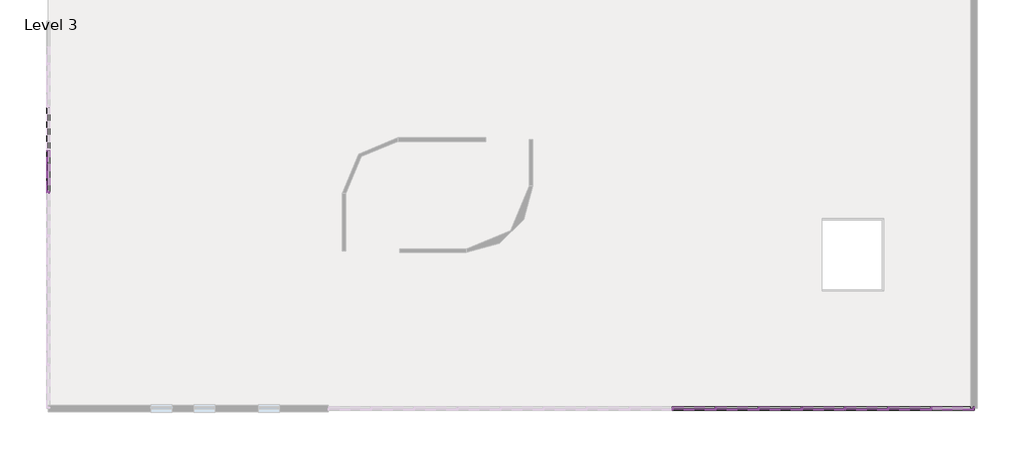
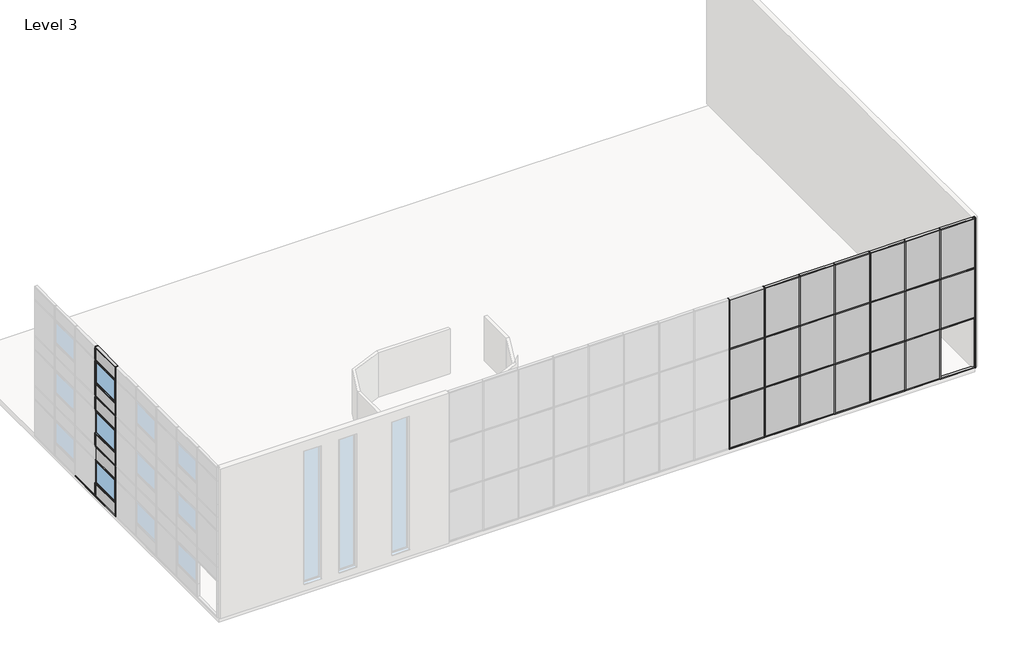
# One storey, part 3 of 5: 77 members, 26 plates, 3 windows.
"""IFC4 building model written with IfcOpenShell, lengths in millimetres."""

import ifcopenshell
import ifcopenshell.guid

model = None  # the IFC model being written
_history = None  # IfcOwnerHistory: only IFC2X3 demands one
_inside = {}  # id of a spatial element -> (the spatial element, [elements in it])
_under = {}  # id of a project, library or spatial element -> (it, [spatial elements below it])
_declared = {}  # id of a project -> (the project, [libraries it declares])
_typed = {}  # id of a type object -> (the type object, [elements of that type])
_made_of = {}  # id of a material, layer set ... -> (it, [elements and type objects made of it])


def new_model(schema):
    """Start an empty IFC model of exactly this schema.

    Asked for "IFC4X3", IfcOpenShell would pick the latest addendum, in which some entities
    have other attributes; the version numbers below select the first issue.
    IFC2X3 requires an IfcOwnerHistory on every rooted entity: one is made here for all.
    """
    global model, _history
    if schema == "IFC4X3":
        model = ifcopenshell.file(schema_version=(4, 3, 0, 0))
    else:
        model = ifcopenshell.file(schema=schema)
    _inside.clear()
    _under.clear()
    _declared.clear()
    _typed.clear()
    _made_of.clear()
    _history = None
    if model.schema == "IFC2X3":
        org = make("IfcOrganization", Name="unknown")
        user = make(
            "IfcPersonAndOrganization",
            ThePerson=make("IfcPerson", FamilyName="unknown"),
            TheOrganization=org,
        )
        app = make(
            "IfcApplication",
            ApplicationDeveloper=org,
            Version="unknown",
            ApplicationFullName="unknown",
            ApplicationIdentifier="unknown",
        )
        _history = make(
            "IfcOwnerHistory",
            OwningUser=user,
            OwningApplication=app,
            ChangeAction="ADDED",
            CreationDate=0,
        )
    return model


def make(cls, **values):
    """One entity of the class cls with the attributes given. An attribute that is None is left unset."""
    return model.create_entity(
        cls, **{name: value for name, value in values.items() if value is not None}
    )


def rooted(cls, **values):
    """An entity with a GlobalId (a new one), such as an element, a storey or a relation."""
    return make(cls, GlobalId=ifcopenshell.guid.new(), OwnerHistory=_history, **values)


def si_unit(unit_type, name, prefix=None):
    """IfcSIUnit, for example si_unit("LENGTHUNIT", "METRE", prefix="MILLI")."""
    return make("IfcSIUnit", UnitType=unit_type, Prefix=prefix, Name=name)


def assignment(units):
    """IfcUnitAssignment: the units of a project."""
    return None if units is None else make("IfcUnitAssignment", Units=units)


def point(xyz):
    """IfcCartesianPoint."""
    return None if xyz is None else make("IfcCartesianPoint", Coordinates=xyz)


def direction(xyz):
    """IfcDirection."""
    return None if xyz is None else make("IfcDirection", DirectionRatios=xyz)


def frame(location, z_axis=None, x_axis=None):
    """IfcAxis2Placement3D, a coordinate frame: its origin and axes. An axis left out is left unset."""
    return make(
        "IfcAxis2Placement3D",
        Location=point(location),
        Axis=direction(z_axis),
        RefDirection=direction(x_axis),
    )


def origin():
    """The frame at (0, 0, 0) with its axes left unset."""
    return frame((0.0, 0.0, 0.0))


def origin_with_axes():
    """The frame at (0, 0, 0) with the z axis (0, 0, 1) and the x axis (1, 0, 0) written out."""
    return frame((0.0, 0.0, 0.0), z_axis=(0.0, 0.0, 1.0), x_axis=(1.0, 0.0, 0.0))


def place(relative_to, where):
    """IfcLocalPlacement: puts the frame where relative to a parent placement (None: the world)."""
    return make(
        "IfcLocalPlacement", PlacementRelTo=relative_to, RelativePlacement=where
    )


def context(
    kind, dimensions, precision=None, world=None, true_north=None, identifier=None
):
    """IfcGeometricRepresentationContext, for example the 3D "Model" context."""
    return make(
        "IfcGeometricRepresentationContext",
        ContextIdentifier=identifier,
        ContextType=kind,
        CoordinateSpaceDimension=dimensions,
        Precision=precision,
        WorldCoordinateSystem=world,
        TrueNorth=true_north,
    )


def project(units=None, contexts=None):
    """IfcProject with its units and contexts."""
    return rooted(
        "IfcProject",
        Name="project",
        RepresentationContexts=contexts,
        UnitsInContext=assignment(units),
    )


def spatial(cls, under=None, at=None, **own):
    """A site, building, storey or space (cls), placed at a placement, below another one or the project."""
    s = rooted(cls, ObjectPlacement=at, **own)
    if under is not None:
        _under.setdefault(under.id(), (under, []))[1].append(s)
    return s


def polyline(points):
    """IfcPolyline through the points."""
    return make("IfcPolyline", Points=[point(p) for p in points])


def outline(outer, holes=None, kind="AREA"):
    """IfcArbitraryClosedProfileDef: a profile drawn as a closed curve; with holes, ...WithVoids."""
    if holes is None:
        return make("IfcArbitraryClosedProfileDef", ProfileType=kind, OuterCurve=outer)
    return make(
        "IfcArbitraryProfileDefWithVoids",
        ProfileType=kind,
        OuterCurve=outer,
        InnerCurves=holes,
    )


def extrude(swept, where, along, depth):
    """IfcExtrudedAreaSolid: the profile swept, set in the frame where, extruded along a direction by depth."""
    return make(
        "IfcExtrudedAreaSolid",
        SweptArea=swept,
        Position=where,
        ExtrudedDirection=direction(along),
        Depth=depth,
    )


def shape(context_of_items, identifier, shape_type, items):
    """IfcShapeRepresentation: the items that make up one representation, for example the "Body"."""
    return make(
        "IfcShapeRepresentation",
        ContextOfItems=context_of_items,
        RepresentationIdentifier=identifier,
        RepresentationType=shape_type,
        Items=items,
    )


def source(mapping_origin, context_of_items, identifier, shape_type, items):
    """IfcRepresentationMap: a shape defined once, which mapped items show again and again."""
    return make(
        "IfcRepresentationMap",
        MappingOrigin=mapping_origin,
        MappedRepresentation=shape(context_of_items, identifier, shape_type, items),
    )


def transform(
    local_origin,
    x_axis=None,
    y_axis=None,
    z_axis=None,
    scale=None,
    scale2=None,
    scale3=None,
    uniform=True,
):
    """IfcCartesianTransformationOperator3D, or its non-uniform kind. x_axis, y_axis, z_axis: its Axis1, 2, 3."""
    if uniform:
        return make(
            "IfcCartesianTransformationOperator3D",
            Axis1=direction(x_axis),
            Axis2=direction(y_axis),
            LocalOrigin=point(local_origin),
            Scale=scale,
            Axis3=direction(z_axis),
        )
    return make(
        "IfcCartesianTransformationOperator3DnonUniform",
        Axis1=direction(x_axis),
        Axis2=direction(y_axis),
        LocalOrigin=point(local_origin),
        Scale=scale,
        Axis3=direction(z_axis),
        Scale2=scale2,
        Scale3=scale3,
    )


def mapped(mapping_source, mapping_target):
    """IfcMappedItem: shows the shape of a source again, moved by a transform."""
    return make(
        "IfcMappedItem", MappingSource=mapping_source, MappingTarget=mapping_target
    )


def made_of(thing, what):
    """Note that an element or type object is made of a material, layer set ...; save() writes the relation."""
    if what is not None:
        _made_of.setdefault(what.id(), (what, []))[1].append(thing)
    return thing


def element(
    cls,
    number,
    at=None,
    inside=None,
    cuts=None,
    type_object=None,
    material=None,
    context=None,
    identifier="Body",
    shape_type=None,
    held_by="IfcProductDefinitionShape",
    body=None,
    shapes=None,
    **own,
):
    """One element of the class cls, such as IfcWall. Its Tag is "e" and its number.

    at: its placement. inside: the storey or other place that contains it. cuts: it is an
    opening in that element (IfcRelVoidsElement). A single representation is given by context,
    identifier, shape_type and body (its items); several are given by shapes. held_by: the class
    of the entity that holds the representations. save() writes the other relations.
    """
    e = rooted(cls, Tag="e%d" % number, ObjectPlacement=at, **own)
    if body is not None:
        shapes = [shape(context, identifier, shape_type, body)]
    if shapes is not None:
        e.Representation = make(held_by, Representations=shapes)
    if inside is not None:
        _inside.setdefault(inside.id(), (inside, []))[1].append(e)
    if cuts is not None:
        rooted(
            "IfcRelVoidsElement", RelatingBuildingElement=cuts, RelatedOpeningElement=e
        )
    if type_object is not None:
        _typed.setdefault(type_object.id(), (type_object, []))[1].append(e)
    return made_of(e, material)


def aggregate(whole, parts):
    """IfcRelAggregates: a whole, such as a stair, and the parts it consists of."""
    return rooted("IfcRelAggregates", RelatingObject=whole, RelatedObjects=parts)


def save(model, path):
    """Write the relations noted so far, then the file.

    IfcRelAggregates (storeys below a building ...), IfcRelContainedInSpatialStructure (elements
    in a storey), IfcRelDefinesByType, IfcRelAssociatesMaterial and IfcRelDeclares: one each for
    every whole, place, type object, material and project.
    """
    for whole, parts in _under.values():
        aggregate(whole, parts)
    for where, things in _inside.values():
        rooted(
            "IfcRelContainedInSpatialStructure",
            RelatedElements=things,
            RelatingStructure=where,
        )
    for kind, things in _typed.values():
        rooted("IfcRelDefinesByType", RelatedObjects=things, RelatingType=kind)
    for what, things in _made_of.values():
        rooted("IfcRelAssociatesMaterial", RelatedObjects=things, RelatingMaterial=what)
    for by, libraries in _declared.values():
        rooted("IfcRelDeclares", RelatingContext=by, RelatedDefinitions=libraries)
    model.write(path)


def rectangular_mullion_50_x_150mm_0967fd3c(model_context):
    return source(origin(), model_context, "Body", "SweptSolid", [
        extrude(outline(polyline([(0.0, 75.0), (0.0, -75.0), (-50.0, -75.0), (-50.0, 75.0), (0.0, 75.0)])), frame((0.0, 0.0, -1950.0000003), z_axis=(0.0, 0.0, 1.0), x_axis=(1.0, 0.0, 0.0)), (0.0, 0.0, 1.0), 1950.0000003),
    ])


def rectangular_mullion_50_x_150mm_f1645b81(model_context):
    return source(origin(), model_context, "Body", "SweptSolid", [
        extrude(outline(polyline([(25.0, 75.0), (25.0, -75.0), (-25.0, -75.0), (-25.0, 75.0), (25.0, 75.0)])), frame((0.0, 0.0, -1950.0000003), z_axis=(0.0, 0.0, 1.0), x_axis=(1.0, 0.0, 0.0)), (0.0, 0.0, 1.0), 1950.0000003),
    ])


def rectangular_mullion_50_x_150mm_14f10ac7(model_context):
    return source(origin(), model_context, "Body", "SweptSolid", [
        extrude(outline(polyline([(25.0, 75.0), (25.0, -75.0), (-25.0, -75.0), (-25.0, 75.0), (25.0, 75.0)])), frame((0.0, 0.0, -800.0), z_axis=(0.0, 0.0, 1.0), x_axis=(1.0, 0.0, 0.0)), (0.0, 0.0, 1.0), 800.0),
    ])


def rectangular_mullion_50_x_150mm_6270d9f9(model_context):
    return source(origin(), model_context, "Body", "SweptSolid", [
        extrude(outline(polyline([(25.0, 75.0), (25.0, -75.0), (-25.0, -75.0), (-25.0, 75.0), (25.0, 75.0)])), frame((0.0, 0.0, -775.0), z_axis=(0.0, 0.0, 1.0), x_axis=(1.0, 0.0, 0.0)), (0.0, 0.0, 1.0), 775.0),
    ])


def rectangular_mullion_50_x_150mm_80d7b263(model_context):
    return source(origin(), model_context, "Body", "SweptSolid", [
        extrude(outline(polyline([(25.0, 75.0), (25.0, -75.0), (-25.0, -75.0), (-25.0, 75.0), (25.0, 75.0)])), frame((0.0, 0.0, -1400.0), z_axis=(0.0, 0.0, 1.0), x_axis=(1.0, 0.0, 0.0)), (0.0, 0.0, 1.0), 1400.0),
    ])


def rectangular_mullion_50_x_150mm_9c26cac3(model_context):
    return source(origin(), model_context, "Body", "SweptSolid", [
        extrude(outline(polyline([(25.0, 75.0), (25.0, -75.0), (-25.0, -75.0), (-25.0, 75.0), (25.0, 75.0)])), frame((0.0, 0.0, -825.0), z_axis=(0.0, 0.0, 1.0), x_axis=(1.0, 0.0, 0.0)), (0.0, 0.0, 1.0), 825.0),
    ])


def rectangular_mullion_50_x_150mm_6c7cb899(model_context):
    return source(origin(), model_context, "Body", "SweptSolid", [
        extrude(outline(polyline([(25.0, 75.0), (25.0, -75.0), (-25.0, -75.0), (-25.0, 75.0), (25.0, 75.0)])), frame((0.0, 0.0, -3000.0), z_axis=(0.0, 0.0, 1.0), x_axis=(1.0, 0.0, 0.0)), (0.0, 0.0, 1.0), 3000.0),
    ])


def rectangular_mullion_50_x_150mm_68c91185(model_context):
    return source(origin(), model_context, "Body", "SweptSolid", [
        extrude(outline(polyline([(0.0, 75.0), (0.0, -75.0), (-50.0, -75.0), (-50.0, 75.0), (0.0, 75.0)])), frame((0.0, 0.0, -3000.0), z_axis=(0.0, 0.0, 1.0), x_axis=(1.0, 0.0, 0.0)), (0.0, 0.0, 1.0), 3000.0),
    ])


def rectangular_mullion_50_x_150mm_7828da58(model_context):
    return source(origin(), model_context, "Body", "SweptSolid", [
        extrude(outline(polyline([(0.0, 75.0), (0.0, -75.0), (-50.0, -75.0), (-50.0, 75.0), (0.0, 75.0)])), frame((0.0, 0.0, -1923.3666669), z_axis=(0.0, 0.0, 1.0), x_axis=(1.0, 0.0, 0.0)), (0.0, 0.0, 1.0), 1923.3666669),
    ])


def rectangular_mullion_50_x_150mm_2c1a111c(model_context):
    return source(origin(), model_context, "Body", "SweptSolid", [
        extrude(outline(polyline([(0.0, 75.0), (0.0, -75.0), (-50.0, -75.0), (-50.0, 75.0), (0.0, 75.0)])), frame((0.0, 0.0, -1948.3666666), z_axis=(0.0, 0.0, 1.0), x_axis=(1.0, 0.0, 0.0)), (0.0, 0.0, 1.0), 1948.3666666),
    ])


def rectangular_mullion_50_x_150mm_6ba4331c(model_context):
    return source(origin(), model_context, "Body", "SweptSolid", [
        extrude(outline(polyline([(25.0, 75.0), (25.0, -75.0), (-25.0, -75.0), (-25.0, 75.0), (25.0, 75.0)])), frame((0.0, 0.0, -1923.3666669), z_axis=(0.0, 0.0, 1.0), x_axis=(1.0, 0.0, 0.0)), (0.0, 0.0, 1.0), 1923.3666669),
    ])


def rectangular_mullion_50_x_150mm_825cde95(model_context):
    return source(origin(), model_context, "Body", "SweptSolid", [
        extrude(outline(polyline([(25.0, 75.0), (25.0, -75.0), (-25.0, -75.0), (-25.0, 75.0), (25.0, 75.0)])), frame((0.0, 0.0, -1948.3666666), z_axis=(0.0, 0.0, 1.0), x_axis=(1.0, 0.0, 0.0)), (0.0, 0.0, 1.0), 1948.3666666),
    ])


def system_panel_glazed_bc1ebc0c(model_context):
    return source(origin(), model_context, "Body", "SweptSolid", [
        extrude(outline(polyline([(975.0000002, 24.5), (-975.0000002, 24.5), (-975.0000002, 49.5), (975.0000002, 49.5), (975.0000002, 24.5)])), origin_with_axes(), (0.0, 0.0, 1.0), 725.0),
    ])


def system_panel_glazed_d82c9dbb(model_context):
    return source(origin(), model_context, "Body", "SweptSolid", [
        extrude(outline(polyline([(975.0000002, 24.5), (-975.0000002, 24.5), (-975.0000002, 49.5), (975.0000002, 49.5), (975.0000002, 24.5)])), origin_with_axes(), (0.0, 0.0, 1.0), 775.0),
    ])


def system_panel_glazed_19a6ddb1(model_context):
    return source(origin(), model_context, "Body", "SweptSolid", [
        extrude(outline(polyline([(961.6833335, 24.5), (-961.6833335, 24.5), (-961.6833335, 49.5), (961.6833335, 49.5), (961.6833335, 24.5)])), origin_with_axes(), (0.0, 0.0, 1.0), 2925.0),
    ])


def system_panel_glazed_e38ee6be(model_context):
    return source(origin(), model_context, "Body", "SweptSolid", [
        extrude(outline(polyline([(974.1833333, 24.5), (-974.1833333, 24.5), (-974.1833333, 49.5), (974.1833333, 49.5), (974.1833333, 24.5)])), origin_with_axes(), (0.0, 0.0, 1.0), 2925.0),
    ])


def system_panel_glazed_cab7de13(model_context):
    return source(origin(), model_context, "Body", "SweptSolid", [
        extrude(outline(polyline([(961.6833335, 24.5), (-961.6833335, 24.5), (-961.6833335, 49.5), (961.6833335, 49.5), (961.6833335, 24.5)])), origin_with_axes(), (0.0, 0.0, 1.0), 2950.0),
    ])


def system_panel_glazed_2cf92cf8(model_context):
    return source(origin(), model_context, "Body", "SweptSolid", [
        extrude(outline(polyline([(974.1833333, 24.5), (-974.1833333, 24.5), (-974.1833333, 49.5), (974.1833333, 49.5), (974.1833333, 24.5)])), origin_with_axes(), (0.0, 0.0, 1.0), 2950.0),
    ])


def m_curtain_wall_awning_m_curtain_wall_awning_db665c81(model_context):
    return source(origin(), model_context, "Body", "SweptSolid", [
        extrude(outline(polyline([(900.0, 44.05), (-900.0, 44.05), (-900.0, 56.75), (900.0, 56.75), (900.0, 44.05)])), frame((0.0, 0.0, 75.0), z_axis=(0.0, 0.0, 1.0), x_axis=(1.0, 0.0, 0.0)), (0.0, 0.0, 1.0), 1200.0),
        extrude(outline(polyline([(1350.0, -975.0), (0.0, -975.0), (0.0, 975.0), (1350.0, 975.0), (1350.0, -975.0)]), holes=[polyline([(1275.0, -900.0), (1275.0, 900.0), (75.0, 900.0), (75.0, -900.0), (1275.0, -900.0)])]), frame((0.0, 25.0, 0.0), z_axis=(0.0, 1.0, 0.0), x_axis=(0.0, 0.0, 1.0)), (0.0, 0.0, 1.0), 50.0),
    ])


model = new_model("IFC4")

# Units and contexts
model_context = context("Model", 3, world=origin())
ifc_project = project(units=[si_unit("LENGTHUNIT", "METRE", prefix="MILLI")], contexts=[model_context])

# Site, building, storey
site = spatial("IfcSite", under=ifc_project)
building = spatial("IfcBuilding", under=site)
storey = spatial("IfcBuildingStorey", under=building, Name="Level 3", Elevation=6000.0)

# Members
placement = place(None, origin())
rectangular_mullion_50_x_150mm_shape = rectangular_mullion_50_x_150mm_0967fd3c(model_context)
element("IfcMember", 1, ObjectType="Rectangular Mullion : 50 x 150mm", at=placement, inside=storey, context=model_context, shape_type="MappedRepresentation", body=[
    mapped(rectangular_mullion_50_x_150mm_shape, transform((-6732.0028633, 48.7577233, 6000.0), x_axis=(0.0, 0.0, -1.0), y_axis=(1.0, 0.0, 0.0), z_axis=(0.0, -1.0, 0.0))),
])
element("IfcMember", 2, ObjectType="Rectangular Mullion : 50 x 150mm", at=placement, inside=storey, context=model_context, shape_type="MappedRepresentation", body=[
    mapped(rectangular_mullion_50_x_150mm_shape, transform((-6732.0028633, 2048.7577233, 6000.0), x_axis=(0.0, 0.0, -1.0), y_axis=(1.0, 0.0, 0.0), z_axis=(0.0, -1.0, 0.0))),
])
rectangular_mullion_50_x_150mm_2_shape = rectangular_mullion_50_x_150mm_f1645b81(model_context)
element("IfcMember", 3, ObjectType="Rectangular Mullion : 50 x 150mm", at=placement, inside=storey, context=model_context, shape_type="MappedRepresentation", body=[
    mapped(rectangular_mullion_50_x_150mm_2_shape, transform((-6732.0028633, 1998.7577233, 14200.0), x_axis=(0.0, 0.0, 1.0), y_axis=(1.0, 0.0, 0.0), z_axis=(0.0, 1.0, 0.0))),
])
element("IfcMember", 4, ObjectType="Rectangular Mullion : 50 x 150mm", at=placement, inside=storey, context=model_context, shape_type="MappedRepresentation", body=[
    mapped(rectangular_mullion_50_x_150mm_2_shape, transform((-6732.0028633, 1998.7577233, 9025.0), x_axis=(0.0, 0.0, 1.0), y_axis=(1.0, 0.0, 0.0), z_axis=(0.0, 1.0, 0.0))),
])
element("IfcMember", 5, ObjectType="Rectangular Mullion : 50 x 150mm", at=placement, inside=storey, context=model_context, shape_type="MappedRepresentation", body=[
    mapped(rectangular_mullion_50_x_150mm_2_shape, transform((-6732.0028633, 1998.7577233, 12025.0), x_axis=(0.0, 0.0, 1.0), y_axis=(1.0, 0.0, 0.0), z_axis=(0.0, 1.0, 0.0))),
])
element("IfcMember", 6, ObjectType="Rectangular Mullion : 50 x 150mm", at=placement, inside=storey, context=model_context, shape_type="MappedRepresentation", body=[
    mapped(rectangular_mullion_50_x_150mm_2_shape, transform((-6732.0028633, 1998.7577233, 12800.0), x_axis=(0.0, 0.0, 1.0), y_axis=(1.0, 0.0, 0.0), z_axis=(0.0, 1.0, 0.0))),
])
element("IfcMember", 7, ObjectType="Rectangular Mullion : 50 x 150mm", at=placement, inside=storey, context=model_context, shape_type="MappedRepresentation", body=[
    mapped(rectangular_mullion_50_x_150mm_2_shape, transform((-6732.0028633, 1998.7577233, 11200.0), x_axis=(0.0, 0.0, 1.0), y_axis=(1.0, 0.0, 0.0), z_axis=(0.0, 1.0, 0.0))),
])
element("IfcMember", 8, ObjectType="Rectangular Mullion : 50 x 150mm", at=placement, inside=storey, context=model_context, shape_type="MappedRepresentation", body=[
    mapped(rectangular_mullion_50_x_150mm_2_shape, transform((-6732.0028633, 1998.7577233, 9800.0), x_axis=(0.0, 0.0, 1.0), y_axis=(1.0, 0.0, 0.0), z_axis=(0.0, 1.0, 0.0))),
])
element("IfcMember", 9, ObjectType="Rectangular Mullion : 50 x 150mm", at=placement, inside=storey, context=model_context, shape_type="MappedRepresentation", body=[
    mapped(rectangular_mullion_50_x_150mm_2_shape, transform((-6732.0028633, 1998.7577233, 8200.0), x_axis=(0.0, 0.0, 1.0), y_axis=(1.0, 0.0, 0.0), z_axis=(0.0, 1.0, 0.0))),
])
element("IfcMember", 10, ObjectType="Rectangular Mullion : 50 x 150mm", at=placement, inside=storey, context=model_context, shape_type="MappedRepresentation", body=[
    mapped(rectangular_mullion_50_x_150mm_2_shape, transform((-6732.0028633, 1998.7577233, 6800.0), x_axis=(0.0, 0.0, 1.0), y_axis=(1.0, 0.0, 0.0), z_axis=(0.0, 1.0, 0.0))),
])
rectangular_mullion_50_x_150mm_3_shape = rectangular_mullion_50_x_150mm_14f10ac7(model_context)
element("IfcMember", 11, ObjectType="Rectangular Mullion : 50 x 150mm", at=placement, inside=storey, context=model_context, shape_type="MappedRepresentation", body=[
    mapped(rectangular_mullion_50_x_150mm_3_shape, transform((-6732.0028633, 23.7577233, 6000.0), x_axis=(0.0, 1.0, 0.0), y_axis=(1.0, 0.0, 0.0), z_axis=(0.0, 0.0, -1.0))),
])
element("IfcMember", 12, ObjectType="Rectangular Mullion : 50 x 150mm", at=placement, inside=storey, context=model_context, shape_type="MappedRepresentation", body=[
    mapped(rectangular_mullion_50_x_150mm_3_shape, transform((-6732.0028633, 2023.7577233, 6000.0), x_axis=(0.0, 1.0, 0.0), y_axis=(1.0, 0.0, 0.0), z_axis=(0.0, 0.0, -1.0))),
])
element("IfcMember", 13, ObjectType="Rectangular Mullion : 50 x 150mm", at=placement, inside=storey, context=model_context, shape_type="MappedRepresentation", body=[
    mapped(rectangular_mullion_50_x_150mm_shape, transform((-6732.0028633, 1998.7577233, 15000.0), x_axis=(0.0, 0.0, 1.0), y_axis=(1.0, 0.0, 0.0), z_axis=(0.0, 1.0, 0.0))),
])
element("IfcMember", 14, ObjectType="Rectangular Mullion : 50 x 150mm", at=placement, inside=storey, context=model_context, shape_type="MappedRepresentation", body=[
    mapped(rectangular_mullion_50_x_150mm_3_shape, transform((-6732.0028633, 23.7577233, 14200.0), x_axis=(0.0, 1.0, 0.0), y_axis=(1.0, 0.0, 0.0), z_axis=(0.0, 0.0, -1.0))),
])
element("IfcMember", 15, ObjectType="Rectangular Mullion : 50 x 150mm", at=placement, inside=storey, context=model_context, shape_type="MappedRepresentation", body=[
    mapped(rectangular_mullion_50_x_150mm_3_shape, transform((-6732.0028633, 2023.7577233, 14200.0), x_axis=(0.0, 1.0, 0.0), y_axis=(1.0, 0.0, 0.0), z_axis=(0.0, 0.0, -1.0))),
])
rectangular_mullion_50_x_150mm_4_shape = rectangular_mullion_50_x_150mm_6270d9f9(model_context)
element("IfcMember", 16, ObjectType="Rectangular Mullion : 50 x 150mm", at=placement, inside=storey, context=model_context, shape_type="MappedRepresentation", body=[
    mapped(rectangular_mullion_50_x_150mm_4_shape, transform((-6732.0028633, 23.7577233, 9025.0), x_axis=(0.0, 1.0, 0.0), y_axis=(1.0, 0.0, 0.0), z_axis=(0.0, 0.0, -1.0))),
])
element("IfcMember", 17, ObjectType="Rectangular Mullion : 50 x 150mm", at=placement, inside=storey, context=model_context, shape_type="MappedRepresentation", body=[
    mapped(rectangular_mullion_50_x_150mm_4_shape, transform((-6732.0028633, 23.7577233, 12025.0), x_axis=(0.0, 1.0, 0.0), y_axis=(1.0, 0.0, 0.0), z_axis=(0.0, 0.0, -1.0))),
])
element("IfcMember", 18, ObjectType="Rectangular Mullion : 50 x 150mm", at=placement, inside=storey, context=model_context, shape_type="MappedRepresentation", body=[
    mapped(rectangular_mullion_50_x_150mm_4_shape, transform((-6732.0028633, 2023.7577233, 9025.0), x_axis=(0.0, 1.0, 0.0), y_axis=(1.0, 0.0, 0.0), z_axis=(0.0, 0.0, -1.0))),
])
element("IfcMember", 19, ObjectType="Rectangular Mullion : 50 x 150mm", at=placement, inside=storey, context=model_context, shape_type="MappedRepresentation", body=[
    mapped(rectangular_mullion_50_x_150mm_4_shape, transform((-6732.0028633, 2023.7577233, 12025.0), x_axis=(0.0, 1.0, 0.0), y_axis=(1.0, 0.0, 0.0), z_axis=(0.0, 0.0, -1.0))),
])
rectangular_mullion_50_x_150mm_5_shape = rectangular_mullion_50_x_150mm_80d7b263(model_context)
element("IfcMember", 20, ObjectType="Rectangular Mullion : 50 x 150mm", at=placement, inside=storey, context=model_context, shape_type="MappedRepresentation", body=[
    mapped(rectangular_mullion_50_x_150mm_5_shape, transform((-6732.0028633, 23.7577233, 12800.0), x_axis=(0.0, 1.0, 0.0), y_axis=(1.0, 0.0, 0.0), z_axis=(0.0, 0.0, -1.0))),
])
element("IfcMember", 21, ObjectType="Rectangular Mullion : 50 x 150mm", at=placement, inside=storey, context=model_context, shape_type="MappedRepresentation", body=[
    mapped(rectangular_mullion_50_x_150mm_5_shape, transform((-6732.0028633, 23.7577233, 9800.0), x_axis=(0.0, 1.0, 0.0), y_axis=(1.0, 0.0, 0.0), z_axis=(0.0, 0.0, -1.0))),
])
element("IfcMember", 22, ObjectType="Rectangular Mullion : 50 x 150mm", at=placement, inside=storey, context=model_context, shape_type="MappedRepresentation", body=[
    mapped(rectangular_mullion_50_x_150mm_5_shape, transform((-6732.0028633, 23.7577233, 6800.0), x_axis=(0.0, 1.0, 0.0), y_axis=(1.0, 0.0, 0.0), z_axis=(0.0, 0.0, -1.0))),
])
element("IfcMember", 23, ObjectType="Rectangular Mullion : 50 x 150mm", at=placement, inside=storey, context=model_context, shape_type="MappedRepresentation", body=[
    mapped(rectangular_mullion_50_x_150mm_5_shape, transform((-6732.0028633, 2023.7577233, 12800.0), x_axis=(0.0, 1.0, 0.0), y_axis=(1.0, 0.0, 0.0), z_axis=(0.0, 0.0, -1.0))),
])
rectangular_mullion_50_x_150mm_6_shape = rectangular_mullion_50_x_150mm_9c26cac3(model_context)
element("IfcMember", 24, ObjectType="Rectangular Mullion : 50 x 150mm", at=placement, inside=storey, context=model_context, shape_type="MappedRepresentation", body=[
    mapped(rectangular_mullion_50_x_150mm_6_shape, transform((-6732.0028633, 23.7577233, 11200.0), x_axis=(0.0, 1.0, 0.0), y_axis=(1.0, 0.0, 0.0), z_axis=(0.0, 0.0, -1.0))),
])
element("IfcMember", 25, ObjectType="Rectangular Mullion : 50 x 150mm", at=placement, inside=storey, context=model_context, shape_type="MappedRepresentation", body=[
    mapped(rectangular_mullion_50_x_150mm_6_shape, transform((-6732.0028633, 23.7577233, 8200.0), x_axis=(0.0, 1.0, 0.0), y_axis=(1.0, 0.0, 0.0), z_axis=(0.0, 0.0, -1.0))),
])
element("IfcMember", 26, ObjectType="Rectangular Mullion : 50 x 150mm", at=placement, inside=storey, context=model_context, shape_type="MappedRepresentation", body=[
    mapped(rectangular_mullion_50_x_150mm_6_shape, transform((-6732.0028633, 2023.7577233, 11200.0), x_axis=(0.0, 1.0, 0.0), y_axis=(1.0, 0.0, 0.0), z_axis=(0.0, 0.0, -1.0))),
])
rectangular_mullion_50_x_150mm_7_shape = rectangular_mullion_50_x_150mm_6c7cb899(model_context)
element("IfcMember", 27, ObjectType="Rectangular Mullion : 50 x 150mm", at=placement, inside=storey, context=model_context, shape_type="MappedRepresentation", body=[
    mapped(rectangular_mullion_50_x_150mm_7_shape, transform((34245.1304697, -10001.242277, 6000.0), x_axis=(-1.0, 0.0, 0.0), y_axis=(0.0, 1.0, 0.0), z_axis=(0.0, 0.0, -1.0))),
])
element("IfcMember", 28, ObjectType="Rectangular Mullion : 50 x 150mm", at=placement, inside=storey, context=model_context, shape_type="MappedRepresentation", body=[
    mapped(rectangular_mullion_50_x_150mm_7_shape, transform((32246.7638031, -10001.242277, 6000.0), x_axis=(-1.0, 0.0, 0.0), y_axis=(0.0, 1.0, 0.0), z_axis=(0.0, 0.0, -1.0))),
])
element("IfcMember", 29, ObjectType="Rectangular Mullion : 50 x 150mm", at=placement, inside=storey, context=model_context, shape_type="MappedRepresentation", body=[
    mapped(rectangular_mullion_50_x_150mm_7_shape, transform((30248.3971365, -10001.242277, 6000.0), x_axis=(-1.0, 0.0, 0.0), y_axis=(0.0, 1.0, 0.0), z_axis=(0.0, 0.0, -1.0))),
])
element("IfcMember", 30, ObjectType="Rectangular Mullion : 50 x 150mm", at=placement, inside=storey, context=model_context, shape_type="MappedRepresentation", body=[
    mapped(rectangular_mullion_50_x_150mm_7_shape, transform((28250.0304699, -10001.242277, 6000.0), x_axis=(-1.0, 0.0, 0.0), y_axis=(0.0, 1.0, 0.0), z_axis=(0.0, 0.0, -1.0))),
])
element("IfcMember", 31, ObjectType="Rectangular Mullion : 50 x 150mm", at=placement, inside=storey, context=model_context, shape_type="MappedRepresentation", body=[
    mapped(rectangular_mullion_50_x_150mm_7_shape, transform((26251.6638032, -10001.242277, 6000.0), x_axis=(-1.0, 0.0, 0.0), y_axis=(0.0, 1.0, 0.0), z_axis=(0.0, 0.0, -1.0))),
])
element("IfcMember", 32, ObjectType="Rectangular Mullion : 50 x 150mm", at=placement, inside=storey, context=model_context, shape_type="MappedRepresentation", body=[
    mapped(rectangular_mullion_50_x_150mm_7_shape, transform((24253.2971366, -10001.242277, 6000.0), x_axis=(-1.0, 0.0, 0.0), y_axis=(0.0, 1.0, 0.0), z_axis=(0.0, 0.0, -1.0))),
])
element("IfcMember", 33, ObjectType="Rectangular Mullion : 50 x 150mm", at=placement, inside=storey, context=model_context, shape_type="MappedRepresentation", body=[
    mapped(rectangular_mullion_50_x_150mm_7_shape, transform((22254.93047, -10001.242277, 6000.0), x_axis=(-1.0, 0.0, 0.0), y_axis=(0.0, 1.0, 0.0), z_axis=(0.0, 0.0, -1.0))),
])
rectangular_mullion_50_x_150mm_8_shape = rectangular_mullion_50_x_150mm_68c91185(model_context)
element("IfcMember", 34, ObjectType="Rectangular Mullion : 50 x 150mm", at=placement, inside=storey, context=model_context, shape_type="MappedRepresentation", body=[
    mapped(rectangular_mullion_50_x_150mm_8_shape, transform((36243.4971367, -10001.242277, 9000.0), x_axis=(1.0, 0.0, 0.0), y_axis=(0.0, 1.0, 0.0), z_axis=(0.0, 0.0, 1.0))),
])
rectangular_mullion_50_x_150mm_9_shape = rectangular_mullion_50_x_150mm_7828da58(model_context)
element("IfcMember", 35, ObjectType="Rectangular Mullion : 50 x 150mm", at=placement, inside=storey, context=model_context, shape_type="MappedRepresentation", body=[
    mapped(rectangular_mullion_50_x_150mm_9_shape, transform((34270.1304697, -10001.242277, 15000.0), x_axis=(0.0, 0.0, 1.0), y_axis=(0.0, 1.0, 0.0), z_axis=(-1.0, 0.0, 0.0))),
])
element("IfcMember", 36, ObjectType="Rectangular Mullion : 50 x 150mm", at=placement, inside=storey, context=model_context, shape_type="MappedRepresentation", body=[
    mapped(rectangular_mullion_50_x_150mm_9_shape, transform((36193.4971367, -10001.242277, 6000.0), x_axis=(0.0, 0.0, -1.0), y_axis=(0.0, 1.0, 0.0), z_axis=(1.0, 0.0, 0.0))),
])
rectangular_mullion_50_x_150mm_10_shape = rectangular_mullion_50_x_150mm_2c1a111c(model_context)
element("IfcMember", 37, ObjectType="Rectangular Mullion : 50 x 150mm", at=placement, inside=storey, context=model_context, shape_type="MappedRepresentation", body=[
    mapped(rectangular_mullion_50_x_150mm_10_shape, transform((32271.7638031, -10001.242277, 15000.0), x_axis=(0.0, 0.0, 1.0), y_axis=(0.0, 1.0, 0.0), z_axis=(-1.0, 0.0, 0.0))),
])
element("IfcMember", 38, ObjectType="Rectangular Mullion : 50 x 150mm", at=placement, inside=storey, context=model_context, shape_type="MappedRepresentation", body=[
    mapped(rectangular_mullion_50_x_150mm_10_shape, transform((30273.3971365, -10001.242277, 15000.0), x_axis=(0.0, 0.0, 1.0), y_axis=(0.0, 1.0, 0.0), z_axis=(-1.0, 0.0, 0.0))),
])
element("IfcMember", 39, ObjectType="Rectangular Mullion : 50 x 150mm", at=placement, inside=storey, context=model_context, shape_type="MappedRepresentation", body=[
    mapped(rectangular_mullion_50_x_150mm_10_shape, transform((28275.0304699, -10001.242277, 15000.0), x_axis=(0.0, 0.0, 1.0), y_axis=(0.0, 1.0, 0.0), z_axis=(-1.0, 0.0, 0.0))),
])
element("IfcMember", 40, ObjectType="Rectangular Mullion : 50 x 150mm", at=placement, inside=storey, context=model_context, shape_type="MappedRepresentation", body=[
    mapped(rectangular_mullion_50_x_150mm_10_shape, transform((26276.6638032, -10001.242277, 15000.0), x_axis=(0.0, 0.0, 1.0), y_axis=(0.0, 1.0, 0.0), z_axis=(-1.0, 0.0, 0.0))),
])
element("IfcMember", 41, ObjectType="Rectangular Mullion : 50 x 150mm", at=placement, inside=storey, context=model_context, shape_type="MappedRepresentation", body=[
    mapped(rectangular_mullion_50_x_150mm_10_shape, transform((24278.2971366, -10001.242277, 15000.0), x_axis=(0.0, 0.0, 1.0), y_axis=(0.0, 1.0, 0.0), z_axis=(-1.0, 0.0, 0.0))),
])
element("IfcMember", 42, ObjectType="Rectangular Mullion : 50 x 150mm", at=placement, inside=storey, context=model_context, shape_type="MappedRepresentation", body=[
    mapped(rectangular_mullion_50_x_150mm_10_shape, transform((34220.1304697, -10001.242277, 6000.0), x_axis=(0.0, 0.0, -1.0), y_axis=(0.0, 1.0, 0.0), z_axis=(1.0, 0.0, 0.0))),
])
element("IfcMember", 43, ObjectType="Rectangular Mullion : 50 x 150mm", at=placement, inside=storey, context=model_context, shape_type="MappedRepresentation", body=[
    mapped(rectangular_mullion_50_x_150mm_10_shape, transform((32221.7638031, -10001.242277, 6000.0), x_axis=(0.0, 0.0, -1.0), y_axis=(0.0, 1.0, 0.0), z_axis=(1.0, 0.0, 0.0))),
])
element("IfcMember", 44, ObjectType="Rectangular Mullion : 50 x 150mm", at=placement, inside=storey, context=model_context, shape_type="MappedRepresentation", body=[
    mapped(rectangular_mullion_50_x_150mm_10_shape, transform((30223.3971365, -10001.242277, 6000.0), x_axis=(0.0, 0.0, -1.0), y_axis=(0.0, 1.0, 0.0), z_axis=(1.0, 0.0, 0.0))),
])
element("IfcMember", 45, ObjectType="Rectangular Mullion : 50 x 150mm", at=placement, inside=storey, context=model_context, shape_type="MappedRepresentation", body=[
    mapped(rectangular_mullion_50_x_150mm_10_shape, transform((28225.0304699, -10001.242277, 6000.0), x_axis=(0.0, 0.0, -1.0), y_axis=(0.0, 1.0, 0.0), z_axis=(1.0, 0.0, 0.0))),
])
element("IfcMember", 46, ObjectType="Rectangular Mullion : 50 x 150mm", at=placement, inside=storey, context=model_context, shape_type="MappedRepresentation", body=[
    mapped(rectangular_mullion_50_x_150mm_10_shape, transform((26226.6638032, -10001.242277, 6000.0), x_axis=(0.0, 0.0, -1.0), y_axis=(0.0, 1.0, 0.0), z_axis=(1.0, 0.0, 0.0))),
])
element("IfcMember", 47, ObjectType="Rectangular Mullion : 50 x 150mm", at=placement, inside=storey, context=model_context, shape_type="MappedRepresentation", body=[
    mapped(rectangular_mullion_50_x_150mm_10_shape, transform((24228.2971366, -10001.242277, 6000.0), x_axis=(0.0, 0.0, -1.0), y_axis=(0.0, 1.0, 0.0), z_axis=(1.0, 0.0, 0.0))),
])
rectangular_mullion_50_x_150mm_11_shape = rectangular_mullion_50_x_150mm_6ba4331c(model_context)
element("IfcMember", 48, ObjectType="Rectangular Mullion : 50 x 150mm", at=placement, inside=storey, context=model_context, shape_type="MappedRepresentation", body=[
    mapped(rectangular_mullion_50_x_150mm_11_shape, transform((34270.1304697, -10001.242277, 9000.0), x_axis=(0.0, 0.0, 1.0), y_axis=(0.0, 1.0, 0.0), z_axis=(-1.0, 0.0, 0.0))),
])
element("IfcMember", 49, ObjectType="Rectangular Mullion : 50 x 150mm", at=placement, inside=storey, context=model_context, shape_type="MappedRepresentation", body=[
    mapped(rectangular_mullion_50_x_150mm_11_shape, transform((34270.1304697, -10001.242277, 12000.0), x_axis=(0.0, 0.0, 1.0), y_axis=(0.0, 1.0, 0.0), z_axis=(-1.0, 0.0, 0.0))),
])
rectangular_mullion_50_x_150mm_12_shape = rectangular_mullion_50_x_150mm_825cde95(model_context)
element("IfcMember", 50, ObjectType="Rectangular Mullion : 50 x 150mm", at=placement, inside=storey, context=model_context, shape_type="MappedRepresentation", body=[
    mapped(rectangular_mullion_50_x_150mm_12_shape, transform((32271.7638031, -10001.242277, 9000.0), x_axis=(0.0, 0.0, 1.0), y_axis=(0.0, 1.0, 0.0), z_axis=(-1.0, 0.0, 0.0))),
])
element("IfcMember", 51, ObjectType="Rectangular Mullion : 50 x 150mm", at=placement, inside=storey, context=model_context, shape_type="MappedRepresentation", body=[
    mapped(rectangular_mullion_50_x_150mm_12_shape, transform((30273.3971365, -10001.242277, 9000.0), x_axis=(0.0, 0.0, 1.0), y_axis=(0.0, 1.0, 0.0), z_axis=(-1.0, 0.0, 0.0))),
])
element("IfcMember", 52, ObjectType="Rectangular Mullion : 50 x 150mm", at=placement, inside=storey, context=model_context, shape_type="MappedRepresentation", body=[
    mapped(rectangular_mullion_50_x_150mm_12_shape, transform((28275.0304699, -10001.242277, 9000.0), x_axis=(0.0, 0.0, 1.0), y_axis=(0.0, 1.0, 0.0), z_axis=(-1.0, 0.0, 0.0))),
])
element("IfcMember", 53, ObjectType="Rectangular Mullion : 50 x 150mm", at=placement, inside=storey, context=model_context, shape_type="MappedRepresentation", body=[
    mapped(rectangular_mullion_50_x_150mm_12_shape, transform((26276.6638032, -10001.242277, 9000.0), x_axis=(0.0, 0.0, 1.0), y_axis=(0.0, 1.0, 0.0), z_axis=(-1.0, 0.0, 0.0))),
])
element("IfcMember", 54, ObjectType="Rectangular Mullion : 50 x 150mm", at=placement, inside=storey, context=model_context, shape_type="MappedRepresentation", body=[
    mapped(rectangular_mullion_50_x_150mm_12_shape, transform((24278.2971366, -10001.242277, 9000.0), x_axis=(0.0, 0.0, 1.0), y_axis=(0.0, 1.0, 0.0), z_axis=(-1.0, 0.0, 0.0))),
])
element("IfcMember", 55, ObjectType="Rectangular Mullion : 50 x 150mm", at=placement, inside=storey, context=model_context, shape_type="MappedRepresentation", body=[
    mapped(rectangular_mullion_50_x_150mm_12_shape, transform((22279.93047, -10001.242277, 9000.0), x_axis=(0.0, 0.0, 1.0), y_axis=(0.0, 1.0, 0.0), z_axis=(-1.0, 0.0, 0.0))),
])
element("IfcMember", 56, ObjectType="Rectangular Mullion : 50 x 150mm", at=placement, inside=storey, context=model_context, shape_type="MappedRepresentation", body=[
    mapped(rectangular_mullion_50_x_150mm_12_shape, transform((32271.7638031, -10001.242277, 12000.0), x_axis=(0.0, 0.0, 1.0), y_axis=(0.0, 1.0, 0.0), z_axis=(-1.0, 0.0, 0.0))),
])
element("IfcMember", 57, ObjectType="Rectangular Mullion : 50 x 150mm", at=placement, inside=storey, context=model_context, shape_type="MappedRepresentation", body=[
    mapped(rectangular_mullion_50_x_150mm_12_shape, transform((30273.3971365, -10001.242277, 12000.0), x_axis=(0.0, 0.0, 1.0), y_axis=(0.0, 1.0, 0.0), z_axis=(-1.0, 0.0, 0.0))),
])
element("IfcMember", 58, ObjectType="Rectangular Mullion : 50 x 150mm", at=placement, inside=storey, context=model_context, shape_type="MappedRepresentation", body=[
    mapped(rectangular_mullion_50_x_150mm_12_shape, transform((28275.0304699, -10001.242277, 12000.0), x_axis=(0.0, 0.0, 1.0), y_axis=(0.0, 1.0, 0.0), z_axis=(-1.0, 0.0, 0.0))),
])
element("IfcMember", 59, ObjectType="Rectangular Mullion : 50 x 150mm", at=placement, inside=storey, context=model_context, shape_type="MappedRepresentation", body=[
    mapped(rectangular_mullion_50_x_150mm_12_shape, transform((26276.6638032, -10001.242277, 12000.0), x_axis=(0.0, 0.0, 1.0), y_axis=(0.0, 1.0, 0.0), z_axis=(-1.0, 0.0, 0.0))),
])
element("IfcMember", 60, ObjectType="Rectangular Mullion : 50 x 150mm", at=placement, inside=storey, context=model_context, shape_type="MappedRepresentation", body=[
    mapped(rectangular_mullion_50_x_150mm_12_shape, transform((24278.2971366, -10001.242277, 12000.0), x_axis=(0.0, 0.0, 1.0), y_axis=(0.0, 1.0, 0.0), z_axis=(-1.0, 0.0, 0.0))),
])
element("IfcMember", 61, ObjectType="Rectangular Mullion : 50 x 150mm", at=placement, inside=storey, context=model_context, shape_type="MappedRepresentation", body=[
    mapped(rectangular_mullion_50_x_150mm_12_shape, transform((22279.93047, -10001.242277, 12000.0), x_axis=(0.0, 0.0, 1.0), y_axis=(0.0, 1.0, 0.0), z_axis=(-1.0, 0.0, 0.0))),
])
element("IfcMember", 62, ObjectType="Rectangular Mullion : 50 x 150mm", at=placement, inside=storey, context=model_context, shape_type="MappedRepresentation", body=[
    mapped(rectangular_mullion_50_x_150mm_7_shape, transform((34245.1304697, -10001.242277, 9000.0), x_axis=(-1.0, 0.0, 0.0), y_axis=(0.0, 1.0, 0.0), z_axis=(0.0, 0.0, -1.0))),
])
element("IfcMember", 63, ObjectType="Rectangular Mullion : 50 x 150mm", at=placement, inside=storey, context=model_context, shape_type="MappedRepresentation", body=[
    mapped(rectangular_mullion_50_x_150mm_7_shape, transform((32246.7638031, -10001.242277, 9000.0), x_axis=(-1.0, 0.0, 0.0), y_axis=(0.0, 1.0, 0.0), z_axis=(0.0, 0.0, -1.0))),
])
element("IfcMember", 64, ObjectType="Rectangular Mullion : 50 x 150mm", at=placement, inside=storey, context=model_context, shape_type="MappedRepresentation", body=[
    mapped(rectangular_mullion_50_x_150mm_7_shape, transform((30248.3971365, -10001.242277, 9000.0), x_axis=(-1.0, 0.0, 0.0), y_axis=(0.0, 1.0, 0.0), z_axis=(0.0, 0.0, -1.0))),
])
element("IfcMember", 65, ObjectType="Rectangular Mullion : 50 x 150mm", at=placement, inside=storey, context=model_context, shape_type="MappedRepresentation", body=[
    mapped(rectangular_mullion_50_x_150mm_7_shape, transform((28250.0304699, -10001.242277, 9000.0), x_axis=(-1.0, 0.0, 0.0), y_axis=(0.0, 1.0, 0.0), z_axis=(0.0, 0.0, -1.0))),
])
element("IfcMember", 66, ObjectType="Rectangular Mullion : 50 x 150mm", at=placement, inside=storey, context=model_context, shape_type="MappedRepresentation", body=[
    mapped(rectangular_mullion_50_x_150mm_7_shape, transform((26251.6638032, -10001.242277, 9000.0), x_axis=(-1.0, 0.0, 0.0), y_axis=(0.0, 1.0, 0.0), z_axis=(0.0, 0.0, -1.0))),
])
element("IfcMember", 67, ObjectType="Rectangular Mullion : 50 x 150mm", at=placement, inside=storey, context=model_context, shape_type="MappedRepresentation", body=[
    mapped(rectangular_mullion_50_x_150mm_7_shape, transform((24253.2971366, -10001.242277, 9000.0), x_axis=(-1.0, 0.0, 0.0), y_axis=(0.0, 1.0, 0.0), z_axis=(0.0, 0.0, -1.0))),
])
element("IfcMember", 68, ObjectType="Rectangular Mullion : 50 x 150mm", at=placement, inside=storey, context=model_context, shape_type="MappedRepresentation", body=[
    mapped(rectangular_mullion_50_x_150mm_7_shape, transform((22254.93047, -10001.242277, 9000.0), x_axis=(-1.0, 0.0, 0.0), y_axis=(0.0, 1.0, 0.0), z_axis=(0.0, 0.0, -1.0))),
])
element("IfcMember", 69, ObjectType="Rectangular Mullion : 50 x 150mm", at=placement, inside=storey, context=model_context, shape_type="MappedRepresentation", body=[
    mapped(rectangular_mullion_50_x_150mm_7_shape, transform((34245.1304697, -10001.242277, 12000.0), x_axis=(-1.0, 0.0, 0.0), y_axis=(0.0, 1.0, 0.0), z_axis=(0.0, 0.0, -1.0))),
])
element("IfcMember", 70, ObjectType="Rectangular Mullion : 50 x 150mm", at=placement, inside=storey, context=model_context, shape_type="MappedRepresentation", body=[
    mapped(rectangular_mullion_50_x_150mm_7_shape, transform((32246.7638031, -10001.242277, 12000.0), x_axis=(-1.0, 0.0, 0.0), y_axis=(0.0, 1.0, 0.0), z_axis=(0.0, 0.0, -1.0))),
])
element("IfcMember", 71, ObjectType="Rectangular Mullion : 50 x 150mm", at=placement, inside=storey, context=model_context, shape_type="MappedRepresentation", body=[
    mapped(rectangular_mullion_50_x_150mm_7_shape, transform((30248.3971365, -10001.242277, 12000.0), x_axis=(-1.0, 0.0, 0.0), y_axis=(0.0, 1.0, 0.0), z_axis=(0.0, 0.0, -1.0))),
])
element("IfcMember", 72, ObjectType="Rectangular Mullion : 50 x 150mm", at=placement, inside=storey, context=model_context, shape_type="MappedRepresentation", body=[
    mapped(rectangular_mullion_50_x_150mm_7_shape, transform((28250.0304699, -10001.242277, 12000.0), x_axis=(-1.0, 0.0, 0.0), y_axis=(0.0, 1.0, 0.0), z_axis=(0.0, 0.0, -1.0))),
])
element("IfcMember", 73, ObjectType="Rectangular Mullion : 50 x 150mm", at=placement, inside=storey, context=model_context, shape_type="MappedRepresentation", body=[
    mapped(rectangular_mullion_50_x_150mm_7_shape, transform((26251.6638032, -10001.242277, 12000.0), x_axis=(-1.0, 0.0, 0.0), y_axis=(0.0, 1.0, 0.0), z_axis=(0.0, 0.0, -1.0))),
])
element("IfcMember", 74, ObjectType="Rectangular Mullion : 50 x 150mm", at=placement, inside=storey, context=model_context, shape_type="MappedRepresentation", body=[
    mapped(rectangular_mullion_50_x_150mm_7_shape, transform((24253.2971366, -10001.242277, 12000.0), x_axis=(-1.0, 0.0, 0.0), y_axis=(0.0, 1.0, 0.0), z_axis=(0.0, 0.0, -1.0))),
])
element("IfcMember", 75, ObjectType="Rectangular Mullion : 50 x 150mm", at=placement, inside=storey, context=model_context, shape_type="MappedRepresentation", body=[
    mapped(rectangular_mullion_50_x_150mm_7_shape, transform((22254.93047, -10001.242277, 12000.0), x_axis=(-1.0, 0.0, 0.0), y_axis=(0.0, 1.0, 0.0), z_axis=(0.0, 0.0, -1.0))),
])
element("IfcMember", 76, ObjectType="Rectangular Mullion : 50 x 150mm", at=placement, inside=storey, context=model_context, shape_type="MappedRepresentation", body=[
    mapped(rectangular_mullion_50_x_150mm_8_shape, transform((36243.4971367, -10001.242277, 15000.0), x_axis=(1.0, 0.0, 0.0), y_axis=(0.0, 1.0, 0.0), z_axis=(0.0, 0.0, 1.0))),
])
element("IfcMember", 77, ObjectType="Rectangular Mullion : 50 x 150mm", at=placement, inside=storey, context=model_context, shape_type="MappedRepresentation", body=[
    mapped(rectangular_mullion_50_x_150mm_8_shape, transform((36243.4971367, -10001.242277, 12000.0), x_axis=(1.0, 0.0, 0.0), y_axis=(0.0, 1.0, 0.0), z_axis=(0.0, 0.0, 1.0))),
])

# Plates
system_panel_glazed_shape = system_panel_glazed_bc1ebc0c(model_context)
element("IfcPlate", 78, ObjectType="System Panel : Glazed", at=placement, inside=storey, context=model_context, shape_type="MappedRepresentation", body=[
    mapped(system_panel_glazed_shape, transform((-6732.0028633, 1023.7577233, 6050.0), x_axis=(0.0, 1.0, 0.0), y_axis=(-1.0, 0.0, 0.0), z_axis=(0.0, 0.0, 1.0))),
])
element("IfcPlate", 79, ObjectType="System Panel : Glazed", at=placement, inside=storey, context=model_context, shape_type="MappedRepresentation", body=[
    mapped(system_panel_glazed_shape, transform((-6732.0028633, 1023.7577233, 14225.0), x_axis=(0.0, 1.0, 0.0), y_axis=(-1.0, 0.0, 0.0), z_axis=(0.0, 0.0, 1.0))),
])
element("IfcPlate", 80, ObjectType="System Panel : Glazed", at=placement, inside=storey, context=model_context, shape_type="MappedRepresentation", body=[
    mapped(system_panel_glazed_shape, transform((-6732.0028633, 1023.7577233, 9050.0), x_axis=(0.0, 1.0, 0.0), y_axis=(-1.0, 0.0, 0.0), z_axis=(0.0, 0.0, 1.0))),
])
element("IfcPlate", 81, ObjectType="System Panel : Glazed", at=placement, inside=storey, context=model_context, shape_type="MappedRepresentation", body=[
    mapped(system_panel_glazed_shape, transform((-6732.0028633, 1023.7577233, 12050.0), x_axis=(0.0, 1.0, 0.0), y_axis=(-1.0, 0.0, 0.0), z_axis=(0.0, 0.0, 1.0))),
])
system_panel_glazed_2_shape = system_panel_glazed_d82c9dbb(model_context)
element("IfcPlate", 82, ObjectType="System Panel : Glazed", at=placement, inside=storey, context=model_context, shape_type="MappedRepresentation", body=[
    mapped(system_panel_glazed_2_shape, transform((-6732.0028633, 1023.7577233, 11225.0), x_axis=(0.0, 1.0, 0.0), y_axis=(-1.0, 0.0, 0.0), z_axis=(0.0, 0.0, 1.0))),
])
element("IfcPlate", 83, ObjectType="System Panel : Glazed", at=placement, inside=storey, context=model_context, shape_type="MappedRepresentation", body=[
    mapped(system_panel_glazed_2_shape, transform((-6732.0028633, 1023.7577233, 8225.0), x_axis=(0.0, 1.0, 0.0), y_axis=(-1.0, 0.0, 0.0), z_axis=(0.0, 0.0, 1.0))),
])
system_panel_glazed_3_shape = system_panel_glazed_19a6ddb1(model_context)
element("IfcPlate", 84, ObjectType="System Panel : Glazed", at=placement, inside=storey, context=model_context, shape_type="MappedRepresentation", body=[
    mapped(system_panel_glazed_3_shape, transform((35231.8138032, -10001.242277, 12025.0), x_axis=(-1.0, 0.0, 0.0), y_axis=(0.0, -1.0, 0.0), z_axis=(0.0, 0.0, 1.0))),
])
system_panel_glazed_4_shape = system_panel_glazed_e38ee6be(model_context)
element("IfcPlate", 85, ObjectType="System Panel : Glazed", at=placement, inside=storey, context=model_context, shape_type="MappedRepresentation", body=[
    mapped(system_panel_glazed_4_shape, transform((33245.9471364, -10001.242277, 6050.0), x_axis=(-1.0, 0.0, 0.0), y_axis=(0.0, -1.0, 0.0), z_axis=(0.0, 0.0, 1.0))),
])
element("IfcPlate", 86, ObjectType="System Panel : Glazed", at=placement, inside=storey, context=model_context, shape_type="MappedRepresentation", body=[
    mapped(system_panel_glazed_4_shape, transform((31247.5804698, -10001.242277, 6050.0), x_axis=(-1.0, 0.0, 0.0), y_axis=(0.0, -1.0, 0.0), z_axis=(0.0, 0.0, 1.0))),
])
element("IfcPlate", 87, ObjectType="System Panel : Glazed", at=placement, inside=storey, context=model_context, shape_type="MappedRepresentation", body=[
    mapped(system_panel_glazed_4_shape, transform((29249.2138032, -10001.242277, 6050.0), x_axis=(-1.0, 0.0, 0.0), y_axis=(0.0, -1.0, 0.0), z_axis=(0.0, 0.0, 1.0))),
])
element("IfcPlate", 88, ObjectType="System Panel : Glazed", at=placement, inside=storey, context=model_context, shape_type="MappedRepresentation", body=[
    mapped(system_panel_glazed_4_shape, transform((27250.8471365, -10001.242277, 6050.0), x_axis=(-1.0, 0.0, 0.0), y_axis=(0.0, -1.0, 0.0), z_axis=(0.0, 0.0, 1.0))),
])
element("IfcPlate", 89, ObjectType="System Panel : Glazed", at=placement, inside=storey, context=model_context, shape_type="MappedRepresentation", body=[
    mapped(system_panel_glazed_4_shape, transform((25252.4804699, -10001.242277, 6050.0), x_axis=(-1.0, 0.0, 0.0), y_axis=(0.0, -1.0, 0.0), z_axis=(0.0, 0.0, 1.0))),
])
element("IfcPlate", 90, ObjectType="System Panel : Glazed", at=placement, inside=storey, context=model_context, shape_type="MappedRepresentation", body=[
    mapped(system_panel_glazed_4_shape, transform((23254.1138033, -10001.242277, 6050.0), x_axis=(-1.0, 0.0, 0.0), y_axis=(0.0, -1.0, 0.0), z_axis=(0.0, 0.0, 1.0))),
])
element("IfcPlate", 91, ObjectType="System Panel : Glazed", at=placement, inside=storey, context=model_context, shape_type="MappedRepresentation", body=[
    mapped(system_panel_glazed_4_shape, transform((33245.9471364, -10001.242277, 12025.0), x_axis=(-1.0, 0.0, 0.0), y_axis=(0.0, -1.0, 0.0), z_axis=(0.0, 0.0, 1.0))),
])
element("IfcPlate", 92, ObjectType="System Panel : Glazed", at=placement, inside=storey, context=model_context, shape_type="MappedRepresentation", body=[
    mapped(system_panel_glazed_4_shape, transform((31247.5804698, -10001.242277, 12025.0), x_axis=(-1.0, 0.0, 0.0), y_axis=(0.0, -1.0, 0.0), z_axis=(0.0, 0.0, 1.0))),
])
element("IfcPlate", 93, ObjectType="System Panel : Glazed", at=placement, inside=storey, context=model_context, shape_type="MappedRepresentation", body=[
    mapped(system_panel_glazed_4_shape, transform((29249.2138032, -10001.242277, 12025.0), x_axis=(-1.0, 0.0, 0.0), y_axis=(0.0, -1.0, 0.0), z_axis=(0.0, 0.0, 1.0))),
])
element("IfcPlate", 94, ObjectType="System Panel : Glazed", at=placement, inside=storey, context=model_context, shape_type="MappedRepresentation", body=[
    mapped(system_panel_glazed_4_shape, transform((27250.8471365, -10001.242277, 12025.0), x_axis=(-1.0, 0.0, 0.0), y_axis=(0.0, -1.0, 0.0), z_axis=(0.0, 0.0, 1.0))),
])
element("IfcPlate", 95, ObjectType="System Panel : Glazed", at=placement, inside=storey, context=model_context, shape_type="MappedRepresentation", body=[
    mapped(system_panel_glazed_4_shape, transform((25252.4804699, -10001.242277, 12025.0), x_axis=(-1.0, 0.0, 0.0), y_axis=(0.0, -1.0, 0.0), z_axis=(0.0, 0.0, 1.0))),
])
element("IfcPlate", 96, ObjectType="System Panel : Glazed", at=placement, inside=storey, context=model_context, shape_type="MappedRepresentation", body=[
    mapped(system_panel_glazed_4_shape, transform((23254.1138033, -10001.242277, 12025.0), x_axis=(-1.0, 0.0, 0.0), y_axis=(0.0, -1.0, 0.0), z_axis=(0.0, 0.0, 1.0))),
])
system_panel_glazed_5_shape = system_panel_glazed_cab7de13(model_context)
element("IfcPlate", 97, ObjectType="System Panel : Glazed", at=placement, inside=storey, context=model_context, shape_type="MappedRepresentation", body=[
    mapped(system_panel_glazed_5_shape, transform((35231.8138032, -10001.242277, 9025.0), x_axis=(-1.0, 0.0, 0.0), y_axis=(0.0, -1.0, 0.0), z_axis=(0.0, 0.0, 1.0))),
])
system_panel_glazed_6_shape = system_panel_glazed_2cf92cf8(model_context)
element("IfcPlate", 98, ObjectType="System Panel : Glazed", at=placement, inside=storey, context=model_context, shape_type="MappedRepresentation", body=[
    mapped(system_panel_glazed_6_shape, transform((33245.9471364, -10001.242277, 9025.0), x_axis=(-1.0, 0.0, 0.0), y_axis=(0.0, -1.0, 0.0), z_axis=(0.0, 0.0, 1.0))),
])
element("IfcPlate", 99, ObjectType="System Panel : Glazed", at=placement, inside=storey, context=model_context, shape_type="MappedRepresentation", body=[
    mapped(system_panel_glazed_6_shape, transform((31247.5804698, -10001.242277, 9025.0), x_axis=(-1.0, 0.0, 0.0), y_axis=(0.0, -1.0, 0.0), z_axis=(0.0, 0.0, 1.0))),
])
element("IfcPlate", 100, ObjectType="System Panel : Glazed", at=placement, inside=storey, context=model_context, shape_type="MappedRepresentation", body=[
    mapped(system_panel_glazed_6_shape, transform((29249.2138032, -10001.242277, 9025.0), x_axis=(-1.0, 0.0, 0.0), y_axis=(0.0, -1.0, 0.0), z_axis=(0.0, 0.0, 1.0))),
])
element("IfcPlate", 101, ObjectType="System Panel : Glazed", at=placement, inside=storey, context=model_context, shape_type="MappedRepresentation", body=[
    mapped(system_panel_glazed_6_shape, transform((27250.8471365, -10001.242277, 9025.0), x_axis=(-1.0, 0.0, 0.0), y_axis=(0.0, -1.0, 0.0), z_axis=(0.0, 0.0, 1.0))),
])
element("IfcPlate", 102, ObjectType="System Panel : Glazed", at=placement, inside=storey, context=model_context, shape_type="MappedRepresentation", body=[
    mapped(system_panel_glazed_6_shape, transform((25252.4804699, -10001.242277, 9025.0), x_axis=(-1.0, 0.0, 0.0), y_axis=(0.0, -1.0, 0.0), z_axis=(0.0, 0.0, 1.0))),
])
element("IfcPlate", 103, ObjectType="System Panel : Glazed", at=placement, inside=storey, context=model_context, shape_type="MappedRepresentation", body=[
    mapped(system_panel_glazed_6_shape, transform((23254.1138033, -10001.242277, 9025.0), x_axis=(-1.0, 0.0, 0.0), y_axis=(0.0, -1.0, 0.0), z_axis=(0.0, 0.0, 1.0))),
])

# Windows
m_curtain_wall_awning_m_curtain_wall_awning_shape = m_curtain_wall_awning_m_curtain_wall_awning_db665c81(model_context)
element("IfcWindow", 104, ObjectType="M_Curtain Wall Awning : M_Curtain Wall Awning", at=placement, inside=storey, context=model_context, shape_type="MappedRepresentation", body=[
    mapped(m_curtain_wall_awning_m_curtain_wall_awning_shape, transform((-6732.0028633, 1023.7577233, 12825.0), x_axis=(0.0, 1.0, 0.0), y_axis=(-1.0, 0.0, 0.0), z_axis=(0.0, 0.0, 1.0))),
])
element("IfcWindow", 105, ObjectType="M_Curtain Wall Awning : M_Curtain Wall Awning", at=placement, inside=storey, context=model_context, shape_type="MappedRepresentation", body=[
    mapped(m_curtain_wall_awning_m_curtain_wall_awning_shape, transform((-6732.0028633, 1023.7577233, 9825.0), x_axis=(0.0, 1.0, 0.0), y_axis=(-1.0, 0.0, 0.0), z_axis=(0.0, 0.0, 1.0))),
])
element("IfcWindow", 106, ObjectType="M_Curtain Wall Awning : M_Curtain Wall Awning", at=placement, inside=storey, context=model_context, shape_type="MappedRepresentation", body=[
    mapped(m_curtain_wall_awning_m_curtain_wall_awning_shape, transform((-6732.0028633, 1023.7577233, 6825.0), x_axis=(0.0, 1.0, 0.0), y_axis=(-1.0, 0.0, 0.0), z_axis=(0.0, 0.0, 1.0))),
])

save(model, "model.ifc")

# Revit data of these elements
# Type "Rectangular Mullion : 50 x 150mm"
#   built-in parameter 1007304 = 0.492126 (stored number, unit not read)
#   built-in parameter 1007301 = 0.082021 (stored number, unit not read)
#   built-in parameter 1007300 = 0.082021 (stored number, unit not read)
# Type "M_Curtain Wall Awning : M_Curtain Wall Awning"
#   Type Mark = "20"
#   Offset = 0.075 m
#   Sash Width = 0.075 m
#   Thickness = 0.050 m
#   Define Thermal Properties by = 1
#   Glass Pane Material = Window - Glass
#   Sash Material = Metal - Aluminum
# Elements 1, 2, 3, 4, 5, 6, 7, 8, 9, 10, 11, 12, 13, 14, 15, 16, 17, 18, 19, 20, 21, 22, 23, 24, 25, 26, 27, 28, 29, 30, 31, 32, 33, 34, 35, 36, 37, 38, 39, 40, 41, 42, 43, 44, 45, 46, 47, 48, 49, 50, 51, 52, 53, 54, 55, 56, 57, 58, 59, 60, 61, 62, 63, 64, 65, 66, 67, 68, 69, 70, 71, 72, 73, 74, 75, 76, 77 (IfcMember, "Rectangular Mullion : 50 x 150mm")
#   Phase Created = New Construction
#   Materials on its faces: "Metal - Aluminium"
# Elements 78, 79, 80, 81, 82, 83, 84, 85, 86, 87, 88, 89, 90, 91, 92, 93, 94, 95, 96, 97, 98, 99, 100, 101, 102, 103 (IfcPlate, "System Panel : Glazed")
#   Phase Created = New Construction
#   Materials on its faces: "Glass"
# Elements 104, 105, 106 (IfcWindow, "M_Curtain Wall Awning : M_Curtain Wall Awning")
#   Phase Created = New Construction
#   Materials on its faces: "Metal - Aluminum", "Window - Glass"
# Materials
#   "Window - Glass": class "Glas", colour RGB 128 128 255, transparency 0.75
#   "Metal - Aluminum": class "Unassigned", colour RGB 247 247 247, transparency 0, Comments = "Rendering appearance not upgraded "
#   "Metal - Aluminium": class "Metal", colour RGB 247 247 247, transparency 0
#   "Glass": class "Glass", colour RGB 0 128 192, transparency 0.9
